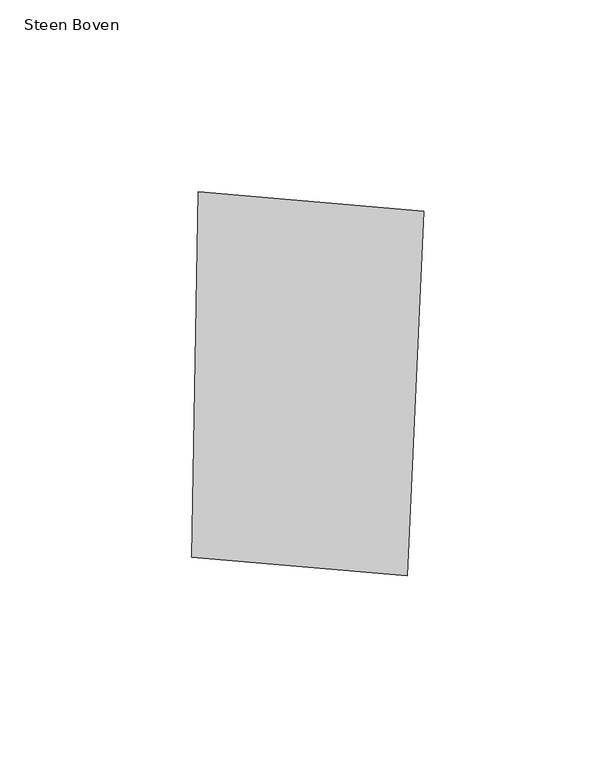
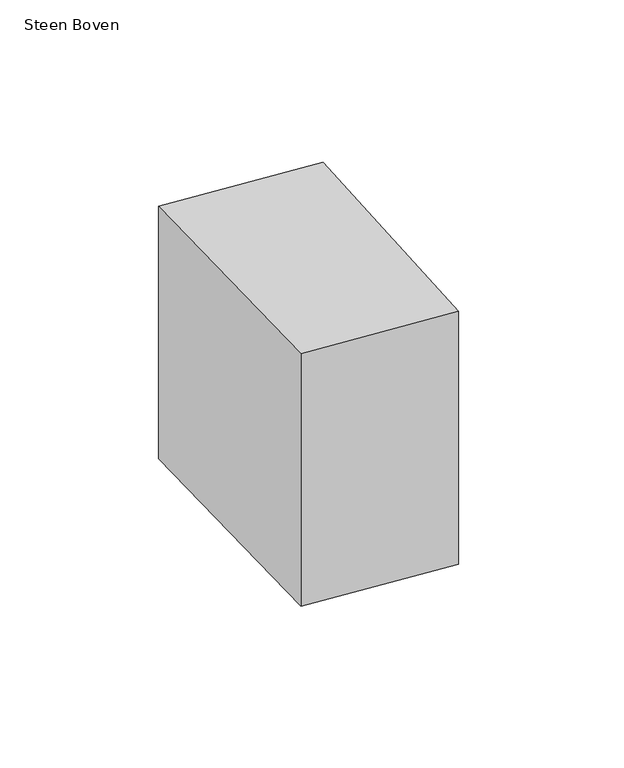
"""IFC4 building model written with IfcOpenShell, lengths in millimetres: proxy geometry, 00_GMA_steen_versie_4 : Steen Boven."""

from ifc_helpers import new_model, si_unit, origin, origin_with_axes, place, context, project, spatial, polyline, outline, extrude, source, transform, mapped, element, save


def steen_boven_1e6de2d0(model_context):
    return source(origin(), model_context, "Body", "SweptSolid", [
        extrude(outline(polyline([(102.7985253, 119.0183414), (98.5670404, 24.026396), (42.4299136, 28.8524186), (44.0502792, 124.0755937), (102.7985253, 119.0183414)])), origin_with_axes(), (0.0, 0.0, 1.0), 100.0),
    ])


if __name__ == "__main__":
    model = new_model("IFC4")
    model_context = context("Model", 3, world=origin())
    ifc_project = project(units=[si_unit("LENGTHUNIT", "METRE", prefix="MILLI")], contexts=[model_context])
    site = spatial("IfcSite", under=ifc_project)
    building = spatial("IfcBuilding", under=site)
    placement = place(None, origin())
    steen_boven_shape = steen_boven_1e6de2d0(model_context)
    element("IfcBuildingElementProxy", 1, Name="00_GMA_steen_versie_4 : Steen Boven", ObjectType="00_GMA_steen_versie_4 : Steen Boven", at=placement, inside=building, context=model_context, shape_type="MappedRepresentation", body=[
        mapped(steen_boven_shape, transform((0.0, 0.0, 0.0), x_axis=(1.0, 0.0, 0.0), y_axis=(0.0, 1.0, 0.0), z_axis=(0.0, 0.0, 1.0))),
    ])
    save(model, "model.ifc")

# Revit data of these elements
# Type "00_GMA_steen_versie_4 : Steen Boven"
#   StootVoegHalfBoven [instance default] = 5 mm
#   StootVoegHalf [instance default] = 5 mm
#   StootVoegBreedteOnder = 10 mm
#   StootVoegBreedteBoven = 10 mm
#   Steendikte = 100 mm
#   LintVoegOnderHalf = 5 mm
#   LintVoegOnder = 10 mm
#   LintVoegBovenHalf = 0 mm
#   LintVoegBoven = 0 mm
#   materiaal = none
#   MateriaalVoeg = none
#   Default Elevation = 0
